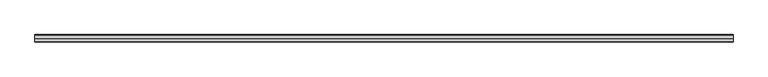
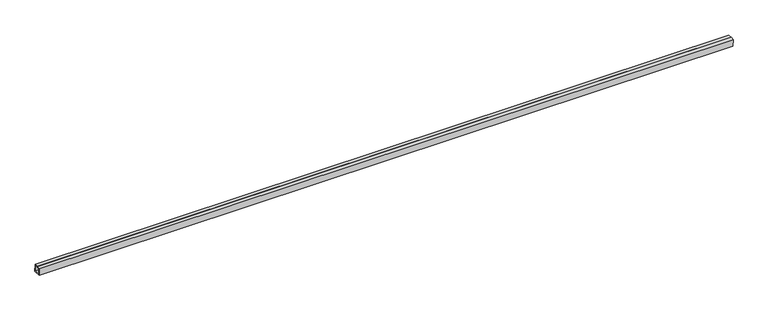
"""IFC4 building model written with IfcOpenShell, lengths in millimetres: proxy geometry, Inner panel:Inner panel:1:Inner panel:1 : Inner panel:Inner panel:300324:2:Inner panel:1:Inner panel:1 : Inner panel:Inner panel:300324:2 : Inner panel:Inner panel:1:Inner panel:1 : Inner panel:Inner panel:300324:300043:49 : Inner panel:Inner panel:1:Inner panel:1 : Inner panel:Inner panel:300324:2:Inner panel:1:Inner panel:1 : Inner panel:Inner panel:300324:2 : Inner panel:Inner panel:1:Inner panel:1 : Inner panel:Inner panel:300324:300043:308120."""

from ifc_helpers import new_model, si_unit, frame, origin, place, context, project, spatial, polyline, outline, extrude, source, transform, mapped, element, save


def generic_models_85e07443(model_context):
    return source(origin(), model_context, "Body", "SweptSolid", [
        extrude(outline(polyline([(-580481.3921913, 3888.2024845), (-580463.1517681, 3888.9625021), (-580461.5656444, 3850.895532), (-580499.6326145, 3849.3094083), (-580501.2187382, 3887.3763783), (-580482.9783151, 3888.136396), (-580482.8791823, 3885.7572103), (-580498.7404199, 3885.0963254), (-580497.3525616, 3851.7877266), (-580464.0439628, 3853.1755849), (-580465.431821, 3886.4841837), (-580481.2930586, 3885.8232988), (-580481.3921913, 3888.2024845)])), frame((664223.0867238, 0.0, 0.0), z_axis=(1.0, 0.0, 0.0), x_axis=(0.0, 1.0, 0.0)), (0.0, 0.0, 1.0), 3657.6),
    ])


if __name__ == "__main__":
    model = new_model("IFC4")
    model_context = context("Model", 3, world=origin())
    ifc_project = project(units=[si_unit("LENGTHUNIT", "METRE", prefix="MILLI")], contexts=[model_context])
    site = spatial("IfcSite", under=ifc_project)
    building = spatial("IfcBuilding", under=site)
    placement = place(None, origin())
    generic_models_shape = generic_models_85e07443(model_context)
    element("IfcBuildingElementProxy", 1, Name="Inner panel:Inner panel:1:Inner panel:1 : Inner panel:Inner panel:300324:2:Inner panel:1:Inner panel:1 : Inner panel:Inner panel:300324:2 : Inner panel:Inner panel:1:Inner panel:1 : Inner panel:Inner panel:300324:300043:49 : Inner panel:Inner panel:1:Inner panel:1 : Inner panel:Inner panel:300324:2:Inner panel:1:Inner panel:1 : Inner panel:Inner panel:300324:2 : Inner panel:Inner panel:1:Inner panel:1 : Inner panel:Inner panel:300324:300043:308120", ObjectType="Inner panel:Inner panel:1:Inner panel:1 : Inner panel:Inner panel:300324:2:Inner panel:1:Inner panel:1 : Inner panel:Inner panel:300324:2 : Inner panel:Inner panel:1:Inner panel:1 : Inner panel:Inner panel:300324:300043:49 : Inner panel:Inner panel:1:Inner panel:1 : Inner panel:Inner panel:300324:2:Inner panel:1:Inner panel:1 : Inner panel:Inner panel:300324:2 : Inner panel:Inner panel:1:Inner panel:1 : Inner panel:Inner panel:300324:300043:308120", at=placement, inside=building, context=model_context, shape_type="MappedRepresentation", body=[
        mapped(generic_models_shape, transform((0.0, 0.0, 0.0), x_axis=(1.0, 0.0, 0.0), y_axis=(0.0, 1.0, 0.0), z_axis=(0.0, 0.0, 1.0))),
    ])
    save(model, "model.ifc")

# Revit data of these elements
# Type "Inner panel:Inner panel:1:Inner panel:1 : Inner panel:Inner panel:300324:2:Inner panel:1:Inner panel:1 : Inner panel:Inner panel:300324:2 : Inner panel:Inner panel:1:Inner panel:1 : Inner panel:Inner panel:300324:300043:49 : Inner panel:Inner panel:1:Inner panel:1 : Inner panel:Inner panel:300324:2:Inner panel:1:Inner panel:1 : Inner panel:Inner panel:300324:2 : Inner panel:Inner panel:1:Inner panel:1 : Inner panel:Inner panel:300324:300043:308120"
#   NameOverride = "Inner panel:Inner panel:1:Inner panel:1 : Inner panel:Inner panel:300324:2:Inner panel:1:Inner panel:1 : Inner panel:Inner panel:300324:2 : Inner panel:Inner panel:1:Inner panel:1 : Inner panel:Inner panel:300324:300043:308120"
#   ObjectTypeOverride = "Inner panel:1:Inner panel:1 : Inner panel:Inner panel:300324:2 : Inner panel:Inner panel:1:Inner panel:1 : Inner panel:Inner panel:300324:300043"
#   Reference = "Inner panel"
#   Tag = "308120"
# Element 1 (IfcBuildingElementProxy, "Inner panel:Inner panel:1:Inner panel:1 : Inner panel:Inner panel:300324:2:Inner panel:1:Inner panel:1 : Inner panel:Inner panel:300324:2 : Inner panel:Inner panel:1:Inner panel:1 : Inner panel:Inner panel:300324:300043:49 : Inner panel:Inner panel:1:Inner panel:1 : Inner panel:Inner panel:300324:2:Inner panel:1:Inner panel:1 : Inner panel:Inner panel:300324:2 : Inner panel:Inner panel:1:Inner panel:1 : Inner panel:Inner panel:300324:300043:308120")
#   Materials on its faces: "1 1/2\" X 1 1/2\" SPLIT-SEAM SQUARE TUBING (~24\" CANTILEVER FROM C.L. OF GLULAM)"
# Materials
#   "1 1/2\" X 1 1/2\" SPLIT-SEAM SQUARE TUBING (~24\" CANTILEVER FROM C.L. OF GLULAM)": class "Unassigned", colour RGB 202 201 200, transparency 0, Cost = 0
